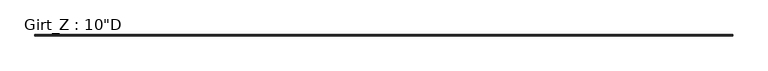
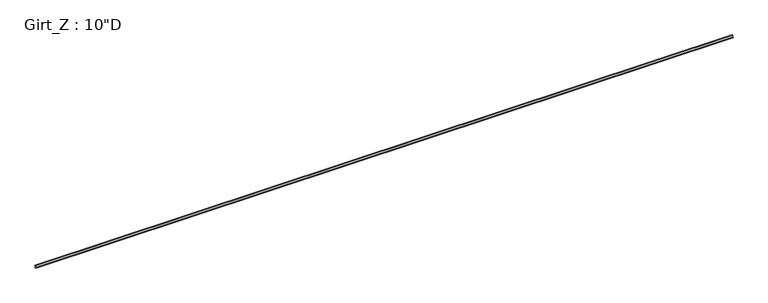
"""IFC4 building model written with IfcOpenShell, lengths in millimetres: beam geometry."""

from ifc_helpers import new_model, si_unit, point, frame, frame_2d, origin, place, context, project, spatial, polyline, circle_curve, trimmed, segment, composite_curve, outline, extrude, source, transform, mapped, element, save


def beam_77f6d86b(model_context):
    return source(origin(), model_context, "Body", "SweptSolid", [
        extrude(outline(composite_curve([segment(polyline([(77.9859375, 127.0), (90.2310415, 112.4068534), (88.1028742, 110.621109), (76.6904765, 124.221875), (3.3005807, 124.221875)]), True, "CONTINUOUS"), segment(trimmed(circle_curve(frame_2d((3.3741066, 122.2381931)), 1.9850441), [point((3.3005807, 124.221875))], [point((1.3890625, 122.2381931))], True, "CARTESIAN"), True, "CONTINUOUS"), segment(polyline([(1.3890625, 122.2381931), (1.3890625, -127.0), (-84.3359375, -127.0), (-96.5810415, -112.4068534), (-94.4528742, -110.621109), (-83.0404765, -124.221875), (-3.2694106, -124.221875)]), True, "CONTINUOUS"), segment(trimmed(circle_curve(frame_2d((-3.3748024, -122.2389339)), 1.9857399), [point((-3.2694106, -124.221875))], [point((-1.3890625, -122.2389339))], True, "CARTESIAN"), True, "CONTINUOUS"), segment(polyline([(-1.3890625, -122.2389339), (-1.3890625, 122.2375)]), True, "CONTINUOUS"), segment(trimmed(circle_curve(frame_2d((3.3734375, 122.2375)), 4.7625), [point((-1.3890625, 122.2375))], [point((3.3734375, 127.0))], False, "CARTESIAN"), True, "CONTINUOUS"), segment(polyline([(3.3734375, 127.0), (77.9859375, 127.0)]), True, "CONTINUOUS")], self_intersect=False)), frame((-44056.3, 0.0, 0.0), z_axis=(1.0, 0.0, 0.0), x_axis=(0.0, 1.0, 0.0)), (0.0, 0.0, 1.0), 88045.925),
    ])


if __name__ == "__main__":
    model = new_model("IFC4")
    model_context = context("Model", 3, world=origin())
    ifc_project = project(units=[si_unit("LENGTHUNIT", "METRE", prefix="MILLI")], contexts=[model_context])
    site = spatial("IfcSite", under=ifc_project)
    building = spatial("IfcBuilding", under=site)
    placement = place(None, origin())
    beam_shape = beam_77f6d86b(model_context)
    element("IfcBeam", 1, ObjectType="Girt_Z : 10\"D", at=placement, inside=building, context=model_context, shape_type="MappedRepresentation", body=[
        mapped(beam_shape, transform((0.0, 0.0, 0.0), x_axis=(1.0, 0.0, 0.0), y_axis=(0.0, 1.0, 0.0), z_axis=(0.0, 0.0, 1.0))),
    ])
    save(model, "model.ifc")

# Revit data of these elements
# Type "Girt_Z : 10\"D"
#   half leg = 0' - 1 11/16"
#   Web_Thickness = 0' - 0 7/64"
#   Length [instance default] = 10' - 0"
#   Leg_2 = 0' - 3 3/8"
#   Leg_1 = 0' - 3 1/8"
#   Height = 0' - 10"
#   Structural Material [instance default] = none
